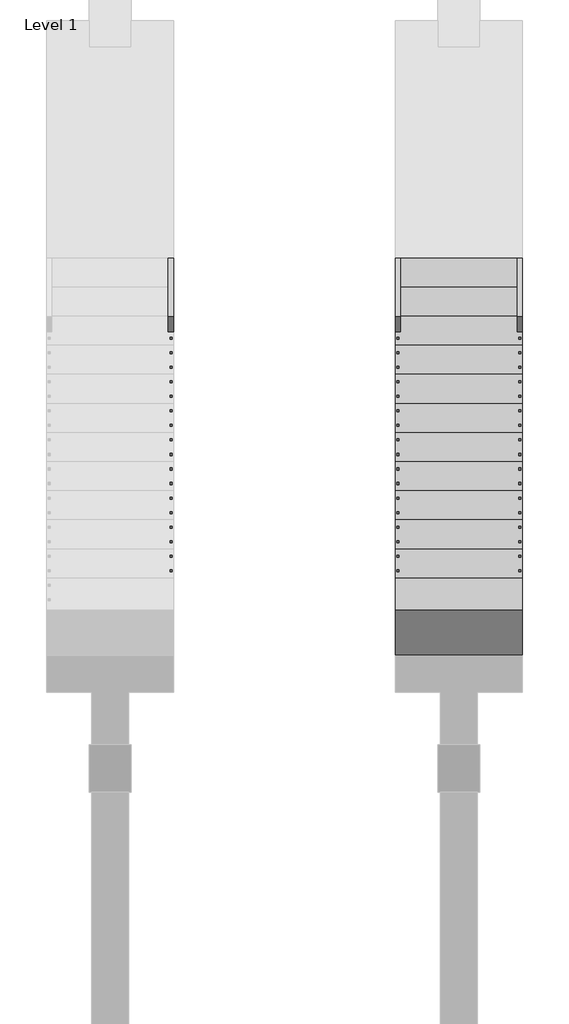
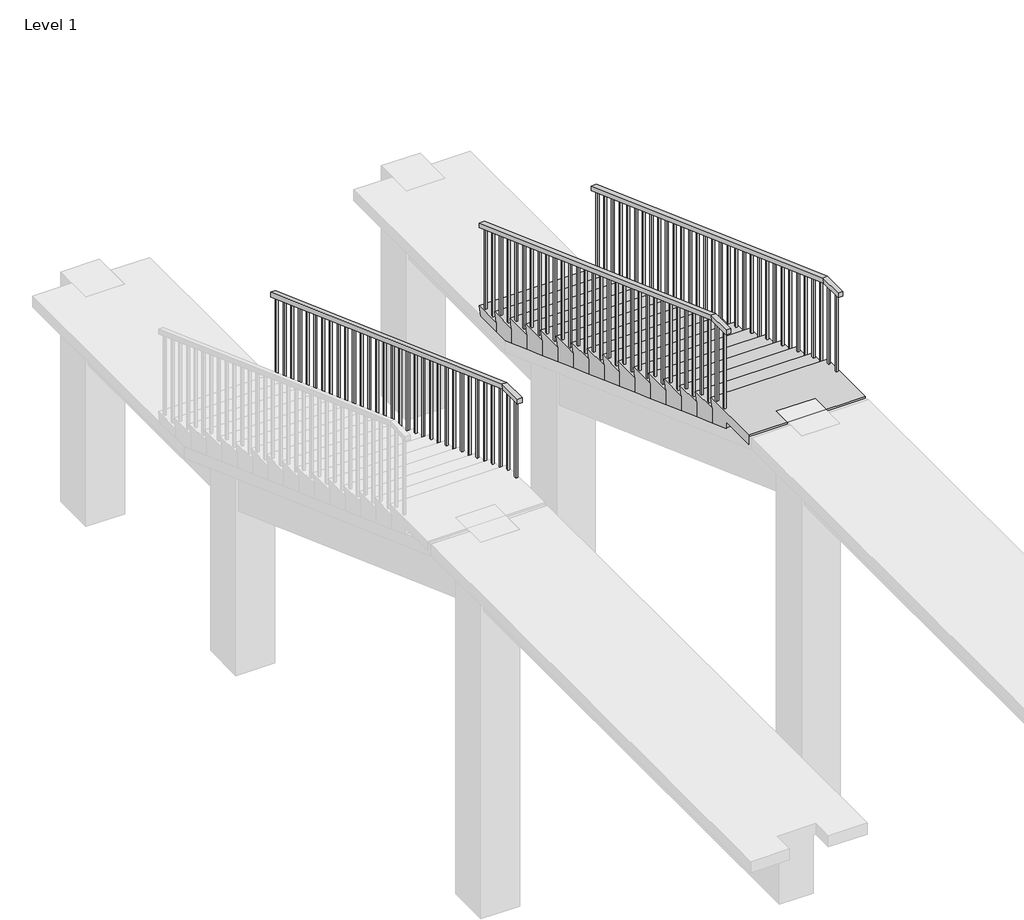
# One storey, part 2 of 2: 3 railings, 1 stair flight.
"""IFC4 building model written with IfcOpenShell, lengths in millimetres."""

from ifc_helpers import new_model, si_unit, frame, origin, place, context, project, spatial, polyline, outline, extrude, faceted_brep, element, save

model = new_model("IFC4")

# Units and contexts
model_context = context("Model", 3, world=origin())
ifc_project = project(units=[si_unit("LENGTHUNIT", "METRE", prefix="MILLI")], contexts=[model_context])

# Site, building, storey
site = spatial("IfcSite", under=ifc_project)
building = spatial("IfcBuilding", under=site)
storey = spatial("IfcBuildingStorey", under=building, Name="Level 1", Elevation=0.0)

# Railings
placement = place(None, origin())
element("IfcRailing", 1, ObjectType="900mm", at=placement, inside=storey, context=model_context, shape_type="SolidModel", body=[
    faceted_brep([(-3859.0267942, 6735.8738053, 1000.0), (-3859.0267942, 6735.8738053, 946.7968186), (-3909.0267942, 6735.8738053, 946.7968186), (-3909.0267942, 6735.8738053, 1000.0), (-3859.0267942, 2610.8738053, 2500.0), (-3859.0267942, 2602.0650564, 2450.0), (-3909.0267942, 2602.0650564, 2450.0), (-3909.0267942, 2610.8738053, 2500.0), (-3859.0267942, 2335.8738053, 2500.0), (-3909.0267942, 2335.8738053, 2500.0), (-3909.0267942, 2335.8738053, 2450.0), (-3859.0267942, 2335.8738053, 2450.0)], [[[0, 1, 2, 3]], [[1, 0, 4, 5]], [[2, 1, 5, 6]], [[3, 2, 6, 7]], [[0, 3, 7, 4]], [[8, 9, 10, 11]], [[5, 4, 8, 11]], [[6, 5, 11, 10]], [[7, 6, 10, 9]], [[4, 7, 9, 8]]]),
    extrude(outline(polyline([(-3894.0267942, 2414.6238053), (-3874.0267942, 2414.6238053), (-3874.0267942, 2394.6238053), (-3894.0267942, 2394.6238053), (-3894.0267942, 2414.6238053)])), frame((0.0, 0.0, 1600.0), z_axis=(0.0, 0.0, 1.0), x_axis=(1.0, 0.0, 0.0)), (0.0, 0.0, 1.0), 850.0),
    extrude(outline(polyline([(-3894.0267942, 2552.1238053), (-3874.0267942, 2552.1238053), (-3874.0267942, 2532.1238053), (-3894.0267942, 2532.1238053), (-3894.0267942, 2552.1238053)])), frame((0.0, 0.0, 1600.0), z_axis=(0.0, 0.0, 1.0), x_axis=(1.0, 0.0, 0.0)), (0.0, 0.0, 1.0), 850.0),
    extrude(outline(polyline([(2689.6238053, 2417.9771109), (2689.6238053, 1500.0), (2669.6238053, 1500.0), (2669.6238053, 2425.3845183), (2689.6238053, 2417.9771109)])), frame((-3894.0267942, 0.0, 0.0), z_axis=(1.0, 0.0, 0.0), x_axis=(0.0, 1.0, 0.0)), (0.0, 0.0, 1.0), 20.0),
    extrude(outline(polyline([(2827.1238053, 2367.9771109), (2827.1238053, 1500.0), (2807.1238053, 1500.0), (2807.1238053, 2375.3845183), (2827.1238053, 2367.9771109)])), frame((-3894.0267942, 0.0, 0.0), z_axis=(1.0, 0.0, 0.0), x_axis=(0.0, 1.0, 0.0)), (0.0, 0.0, 1.0), 20.0),
    extrude(outline(polyline([(2964.6238053, 2317.9771109), (2964.6238053, 1400.0), (2944.6238053, 1400.0), (2944.6238053, 2325.3845183), (2964.6238053, 2317.9771109)])), frame((-3894.0267942, 0.0, 0.0), z_axis=(1.0, 0.0, 0.0), x_axis=(0.0, 1.0, 0.0)), (0.0, 0.0, 1.0), 20.0),
    extrude(outline(polyline([(3102.1238053, 2267.9771109), (3102.1238053, 1400.0), (3082.1238053, 1400.0), (3082.1238053, 2275.3845183), (3102.1238053, 2267.9771109)])), frame((-3894.0267942, 0.0, 0.0), z_axis=(1.0, 0.0, 0.0), x_axis=(0.0, 1.0, 0.0)), (0.0, 0.0, 1.0), 20.0),
    extrude(outline(polyline([(3239.6238053, 2217.9771109), (3239.6238053, 1300.0), (3219.6238053, 1300.0), (3219.6238053, 2225.3845183), (3239.6238053, 2217.9771109)])), frame((-3894.0267942, 0.0, 0.0), z_axis=(1.0, 0.0, 0.0), x_axis=(0.0, 1.0, 0.0)), (0.0, 0.0, 1.0), 20.0),
    extrude(outline(polyline([(3377.1238053, 2167.9771109), (3377.1238053, 1300.0), (3357.1238053, 1300.0), (3357.1238053, 2175.3845183), (3377.1238053, 2167.9771109)])), frame((-3894.0267942, 0.0, 0.0), z_axis=(1.0, 0.0, 0.0), x_axis=(0.0, 1.0, 0.0)), (0.0, 0.0, 1.0), 20.0),
    extrude(outline(polyline([(3514.6238053, 2117.9771109), (3514.6238053, 1200.0), (3494.6238053, 1200.0), (3494.6238053, 2125.3845183), (3514.6238053, 2117.9771109)])), frame((-3894.0267942, 0.0, 0.0), z_axis=(1.0, 0.0, 0.0), x_axis=(0.0, 1.0, 0.0)), (0.0, 0.0, 1.0), 20.0),
    extrude(outline(polyline([(3652.1238053, 2067.9771109), (3652.1238053, 1200.0), (3632.1238053, 1200.0), (3632.1238053, 2075.3845183), (3652.1238053, 2067.9771109)])), frame((-3894.0267942, 0.0, 0.0), z_axis=(1.0, 0.0, 0.0), x_axis=(0.0, 1.0, 0.0)), (0.0, 0.0, 1.0), 20.0),
    extrude(outline(polyline([(3789.6238053, 2017.9771109), (3789.6238053, 1100.0), (3769.6238053, 1100.0), (3769.6238053, 2025.3845183), (3789.6238053, 2017.9771109)])), frame((-3894.0267942, 0.0, 0.0), z_axis=(1.0, 0.0, 0.0), x_axis=(0.0, 1.0, 0.0)), (0.0, 0.0, 1.0), 20.0),
    extrude(outline(polyline([(3927.1238053, 1967.9771109), (3927.1238053, 1100.0), (3907.1238053, 1100.0), (3907.1238053, 1975.3845183), (3927.1238053, 1967.9771109)])), frame((-3894.0267942, 0.0, 0.0), z_axis=(1.0, 0.0, 0.0), x_axis=(0.0, 1.0, 0.0)), (0.0, 0.0, 1.0), 20.0),
    extrude(outline(polyline([(4064.6238053, 1917.9771109), (4064.6238053, 1000.0), (4044.6238053, 1000.0), (4044.6238053, 1925.3845183), (4064.6238053, 1917.9771109)])), frame((-3894.0267942, 0.0, 0.0), z_axis=(1.0, 0.0, 0.0), x_axis=(0.0, 1.0, 0.0)), (0.0, 0.0, 1.0), 20.0),
    extrude(outline(polyline([(4202.1238053, 1867.9771109), (4202.1238053, 1000.0), (4182.1238053, 1000.0), (4182.1238053, 1875.3845183), (4202.1238053, 1867.9771109)])), frame((-3894.0267942, 0.0, 0.0), z_axis=(1.0, 0.0, 0.0), x_axis=(0.0, 1.0, 0.0)), (0.0, 0.0, 1.0), 20.0),
    extrude(outline(polyline([(4339.6238053, 1817.9771109), (4339.6238053, 900.0), (4319.6238053, 900.0), (4319.6238053, 1825.3845183), (4339.6238053, 1817.9771109)])), frame((-3894.0267942, 0.0, 0.0), z_axis=(1.0, 0.0, 0.0), x_axis=(0.0, 1.0, 0.0)), (0.0, 0.0, 1.0), 20.0),
    extrude(outline(polyline([(4477.1238053, 1767.9771109), (4477.1238053, 900.0), (4457.1238053, 900.0), (4457.1238053, 1775.3845183), (4477.1238053, 1767.9771109)])), frame((-3894.0267942, 0.0, 0.0), z_axis=(1.0, 0.0, 0.0), x_axis=(0.0, 1.0, 0.0)), (0.0, 0.0, 1.0), 20.0),
    extrude(outline(polyline([(4614.6238053, 1717.9771109), (4614.6238053, 800.0), (4594.6238053, 800.0), (4594.6238053, 1725.3845183), (4614.6238053, 1717.9771109)])), frame((-3894.0267942, 0.0, 0.0), z_axis=(1.0, 0.0, 0.0), x_axis=(0.0, 1.0, 0.0)), (0.0, 0.0, 1.0), 20.0),
    extrude(outline(polyline([(4752.1238053, 1667.9771109), (4752.1238053, 800.0), (4732.1238053, 800.0), (4732.1238053, 1675.3845183), (4752.1238053, 1667.9771109)])), frame((-3894.0267942, 0.0, 0.0), z_axis=(1.0, 0.0, 0.0), x_axis=(0.0, 1.0, 0.0)), (0.0, 0.0, 1.0), 20.0),
    extrude(outline(polyline([(4889.6238053, 1617.9771109), (4889.6238053, 700.0), (4869.6238053, 700.0), (4869.6238053, 1625.3845183), (4889.6238053, 1617.9771109)])), frame((-3894.0267942, 0.0, 0.0), z_axis=(1.0, 0.0, 0.0), x_axis=(0.0, 1.0, 0.0)), (0.0, 0.0, 1.0), 20.0),
    extrude(outline(polyline([(5027.1238053, 1567.9771109), (5027.1238053, 700.0), (5007.1238053, 700.0), (5007.1238053, 1575.3845183), (5027.1238053, 1567.9771109)])), frame((-3894.0267942, 0.0, 0.0), z_axis=(1.0, 0.0, 0.0), x_axis=(0.0, 1.0, 0.0)), (0.0, 0.0, 1.0), 20.0),
    extrude(outline(polyline([(5164.6238053, 1517.9771109), (5164.6238053, 600.0), (5144.6238053, 600.0), (5144.6238053, 1525.3845183), (5164.6238053, 1517.9771109)])), frame((-3894.0267942, 0.0, 0.0), z_axis=(1.0, 0.0, 0.0), x_axis=(0.0, 1.0, 0.0)), (0.0, 0.0, 1.0), 20.0),
    extrude(outline(polyline([(5302.1238053, 1467.9771109), (5302.1238053, 600.0), (5282.1238053, 600.0), (5282.1238053, 1475.3845183), (5302.1238053, 1467.9771109)])), frame((-3894.0267942, 0.0, 0.0), z_axis=(1.0, 0.0, 0.0), x_axis=(0.0, 1.0, 0.0)), (0.0, 0.0, 1.0), 20.0),
    extrude(outline(polyline([(5439.6238053, 1417.9771109), (5439.6238053, 500.0), (5419.6238053, 500.0), (5419.6238053, 1425.3845183), (5439.6238053, 1417.9771109)])), frame((-3894.0267942, 0.0, 0.0), z_axis=(1.0, 0.0, 0.0), x_axis=(0.0, 1.0, 0.0)), (0.0, 0.0, 1.0), 20.0),
    extrude(outline(polyline([(5577.1238053, 1367.9771109), (5577.1238053, 500.0), (5557.1238053, 500.0), (5557.1238053, 1375.3845183), (5577.1238053, 1367.9771109)])), frame((-3894.0267942, 0.0, 0.0), z_axis=(1.0, 0.0, 0.0), x_axis=(0.0, 1.0, 0.0)), (0.0, 0.0, 1.0), 20.0),
    extrude(outline(polyline([(5714.6238053, 1317.9771109), (5714.6238053, 400.0), (5694.6238053, 400.0), (5694.6238053, 1325.3845183), (5714.6238053, 1317.9771109)])), frame((-3894.0267942, 0.0, 0.0), z_axis=(1.0, 0.0, 0.0), x_axis=(0.0, 1.0, 0.0)), (0.0, 0.0, 1.0), 20.0),
    extrude(outline(polyline([(5852.1238053, 1267.9771109), (5852.1238053, 400.0), (5832.1238053, 400.0), (5832.1238053, 1275.3845183), (5852.1238053, 1267.9771109)])), frame((-3894.0267942, 0.0, 0.0), z_axis=(1.0, 0.0, 0.0), x_axis=(0.0, 1.0, 0.0)), (0.0, 0.0, 1.0), 20.0),
    extrude(outline(polyline([(5989.6238053, 1217.9771109), (5989.6238053, 300.0), (5969.6238053, 300.0), (5969.6238053, 1225.3845183), (5989.6238053, 1217.9771109)])), frame((-3894.0267942, 0.0, 0.0), z_axis=(1.0, 0.0, 0.0), x_axis=(0.0, 1.0, 0.0)), (0.0, 0.0, 1.0), 20.0),
    extrude(outline(polyline([(6127.1238053, 1167.9771109), (6127.1238053, 300.0), (6107.1238053, 300.0), (6107.1238053, 1175.3845183), (6127.1238053, 1167.9771109)])), frame((-3894.0267942, 0.0, 0.0), z_axis=(1.0, 0.0, 0.0), x_axis=(0.0, 1.0, 0.0)), (0.0, 0.0, 1.0), 20.0),
    extrude(outline(polyline([(6264.6238053, 1117.9771109), (6264.6238053, 200.0), (6244.6238053, 200.0), (6244.6238053, 1125.3845183), (6264.6238053, 1117.9771109)])), frame((-3894.0267942, 0.0, 0.0), z_axis=(1.0, 0.0, 0.0), x_axis=(0.0, 1.0, 0.0)), (0.0, 0.0, 1.0), 20.0),
    extrude(outline(polyline([(6402.1238053, 1067.9771109), (6402.1238053, 200.0), (6382.1238053, 200.0), (6382.1238053, 1075.3845183), (6402.1238053, 1067.9771109)])), frame((-3894.0267942, 0.0, 0.0), z_axis=(1.0, 0.0, 0.0), x_axis=(0.0, 1.0, 0.0)), (0.0, 0.0, 1.0), 20.0),
    extrude(outline(polyline([(6539.6238053, 1017.9771109), (6539.6238053, 100.0), (6519.6238053, 100.0), (6519.6238053, 1025.3845183), (6539.6238053, 1017.9771109)])), frame((-3894.0267942, 0.0, 0.0), z_axis=(1.0, 0.0, 0.0), x_axis=(0.0, 1.0, 0.0)), (0.0, 0.0, 1.0), 20.0),
    extrude(outline(polyline([(6677.1238053, 967.9771109), (6677.1238053, 100.0), (6657.1238053, 100.0), (6657.1238053, 975.3845183), (6677.1238053, 967.9771109)])), frame((-3894.0267942, 0.0, 0.0), z_axis=(1.0, 0.0, 0.0), x_axis=(0.0, 1.0, 0.0)), (0.0, 0.0, 1.0), 20.0),
])
element("IfcRailing", 2, ObjectType="900mm", at=placement, inside=storey, context=model_context, shape_type="SolidModel", body=[
    faceted_brep([(-2706.8056398, 6735.8738053, 1000.0), (-2706.8056398, 6735.8738053, 946.7968186), (-2756.8056398, 6735.8738053, 946.7968186), (-2756.8056398, 6735.8738053, 1000.0), (-2706.8056398, 2610.8738053, 2500.0), (-2706.8056398, 2602.0650564, 2450.0), (-2756.8056398, 2602.0650564, 2450.0), (-2756.8056398, 2610.8738053, 2500.0), (-2706.8056398, 2335.8738053, 2500.0), (-2756.8056398, 2335.8738053, 2500.0), (-2756.8056398, 2335.8738053, 2450.0), (-2706.8056398, 2335.8738053, 2450.0)], [[[0, 1, 2, 3]], [[1, 0, 4, 5]], [[2, 1, 5, 6]], [[3, 2, 6, 7]], [[0, 3, 7, 4]], [[8, 9, 10, 11]], [[5, 4, 8, 11]], [[6, 5, 11, 10]], [[7, 6, 10, 9]], [[4, 7, 9, 8]]]),
    extrude(outline(polyline([(-2721.8056398, 2414.6238053), (-2721.8056398, 2394.6238053), (-2741.8056398, 2394.6238053), (-2741.8056398, 2414.6238053), (-2721.8056398, 2414.6238053)])), frame((0.0, 0.0, 1600.0), z_axis=(0.0, 0.0, 1.0), x_axis=(1.0, 0.0, 0.0)), (0.0, 0.0, 1.0), 850.0),
    extrude(outline(polyline([(-2721.8056398, 2552.1238053), (-2721.8056398, 2532.1238053), (-2741.8056398, 2532.1238053), (-2741.8056398, 2552.1238053), (-2721.8056398, 2552.1238053)])), frame((0.0, 0.0, 1600.0), z_axis=(0.0, 0.0, 1.0), x_axis=(1.0, 0.0, 0.0)), (0.0, 0.0, 1.0), 850.0),
    extrude(outline(polyline([(2689.6238053, 1500.0), (2669.6238053, 1500.0), (2669.6238053, 2425.3845183), (2689.6238053, 2417.9771109), (2689.6238053, 1500.0)])), frame((-2741.8056398, 0.0, 0.0), z_axis=(1.0, 0.0, 0.0), x_axis=(0.0, 1.0, 0.0)), (0.0, 0.0, 1.0), 20.0),
    extrude(outline(polyline([(2827.1238053, 1500.0), (2807.1238053, 1500.0), (2807.1238053, 2375.3845183), (2827.1238053, 2367.9771109), (2827.1238053, 1500.0)])), frame((-2741.8056398, 0.0, 0.0), z_axis=(1.0, 0.0, 0.0), x_axis=(0.0, 1.0, 0.0)), (0.0, 0.0, 1.0), 20.0),
    extrude(outline(polyline([(2964.6238053, 1400.0), (2944.6238053, 1400.0), (2944.6238053, 2325.3845183), (2964.6238053, 2317.9771109), (2964.6238053, 1400.0)])), frame((-2741.8056398, 0.0, 0.0), z_axis=(1.0, 0.0, 0.0), x_axis=(0.0, 1.0, 0.0)), (0.0, 0.0, 1.0), 20.0),
    extrude(outline(polyline([(3102.1238053, 1400.0), (3082.1238053, 1400.0), (3082.1238053, 2275.3845183), (3102.1238053, 2267.9771109), (3102.1238053, 1400.0)])), frame((-2741.8056398, 0.0, 0.0), z_axis=(1.0, 0.0, 0.0), x_axis=(0.0, 1.0, 0.0)), (0.0, 0.0, 1.0), 20.0),
    extrude(outline(polyline([(3239.6238053, 1300.0), (3219.6238053, 1300.0), (3219.6238053, 2225.3845183), (3239.6238053, 2217.9771109), (3239.6238053, 1300.0)])), frame((-2741.8056398, 0.0, 0.0), z_axis=(1.0, 0.0, 0.0), x_axis=(0.0, 1.0, 0.0)), (0.0, 0.0, 1.0), 20.0),
    extrude(outline(polyline([(3377.1238053, 1300.0), (3357.1238053, 1300.0), (3357.1238053, 2175.3845183), (3377.1238053, 2167.9771109), (3377.1238053, 1300.0)])), frame((-2741.8056398, 0.0, 0.0), z_axis=(1.0, 0.0, 0.0), x_axis=(0.0, 1.0, 0.0)), (0.0, 0.0, 1.0), 20.0),
    extrude(outline(polyline([(3514.6238053, 1200.0), (3494.6238053, 1200.0), (3494.6238053, 2125.3845183), (3514.6238053, 2117.9771109), (3514.6238053, 1200.0)])), frame((-2741.8056398, 0.0, 0.0), z_axis=(1.0, 0.0, 0.0), x_axis=(0.0, 1.0, 0.0)), (0.0, 0.0, 1.0), 20.0),
    extrude(outline(polyline([(3652.1238053, 1200.0), (3632.1238053, 1200.0), (3632.1238053, 2075.3845183), (3652.1238053, 2067.9771109), (3652.1238053, 1200.0)])), frame((-2741.8056398, 0.0, 0.0), z_axis=(1.0, 0.0, 0.0), x_axis=(0.0, 1.0, 0.0)), (0.0, 0.0, 1.0), 20.0),
    extrude(outline(polyline([(3789.6238053, 1100.0), (3769.6238053, 1100.0), (3769.6238053, 2025.3845183), (3789.6238053, 2017.9771109), (3789.6238053, 1100.0)])), frame((-2741.8056398, 0.0, 0.0), z_axis=(1.0, 0.0, 0.0), x_axis=(0.0, 1.0, 0.0)), (0.0, 0.0, 1.0), 20.0),
    extrude(outline(polyline([(3927.1238053, 1100.0), (3907.1238053, 1100.0), (3907.1238053, 1975.3845183), (3927.1238053, 1967.9771109), (3927.1238053, 1100.0)])), frame((-2741.8056398, 0.0, 0.0), z_axis=(1.0, 0.0, 0.0), x_axis=(0.0, 1.0, 0.0)), (0.0, 0.0, 1.0), 20.0),
    extrude(outline(polyline([(4064.6238053, 1000.0), (4044.6238053, 1000.0), (4044.6238053, 1925.3845183), (4064.6238053, 1917.9771109), (4064.6238053, 1000.0)])), frame((-2741.8056398, 0.0, 0.0), z_axis=(1.0, 0.0, 0.0), x_axis=(0.0, 1.0, 0.0)), (0.0, 0.0, 1.0), 20.0),
    extrude(outline(polyline([(4202.1238053, 1000.0), (4182.1238053, 1000.0), (4182.1238053, 1875.3845183), (4202.1238053, 1867.9771109), (4202.1238053, 1000.0)])), frame((-2741.8056398, 0.0, 0.0), z_axis=(1.0, 0.0, 0.0), x_axis=(0.0, 1.0, 0.0)), (0.0, 0.0, 1.0), 20.0),
    extrude(outline(polyline([(4339.6238053, 900.0), (4319.6238053, 900.0), (4319.6238053, 1825.3845183), (4339.6238053, 1817.9771109), (4339.6238053, 900.0)])), frame((-2741.8056398, 0.0, 0.0), z_axis=(1.0, 0.0, 0.0), x_axis=(0.0, 1.0, 0.0)), (0.0, 0.0, 1.0), 20.0),
    extrude(outline(polyline([(4477.1238053, 900.0), (4457.1238053, 900.0), (4457.1238053, 1775.3845183), (4477.1238053, 1767.9771109), (4477.1238053, 900.0)])), frame((-2741.8056398, 0.0, 0.0), z_axis=(1.0, 0.0, 0.0), x_axis=(0.0, 1.0, 0.0)), (0.0, 0.0, 1.0), 20.0),
    extrude(outline(polyline([(4614.6238053, 800.0), (4594.6238053, 800.0), (4594.6238053, 1725.3845183), (4614.6238053, 1717.9771109), (4614.6238053, 800.0)])), frame((-2741.8056398, 0.0, 0.0), z_axis=(1.0, 0.0, 0.0), x_axis=(0.0, 1.0, 0.0)), (0.0, 0.0, 1.0), 20.0),
    extrude(outline(polyline([(4752.1238053, 800.0), (4732.1238053, 800.0), (4732.1238053, 1675.3845183), (4752.1238053, 1667.9771109), (4752.1238053, 800.0)])), frame((-2741.8056398, 0.0, 0.0), z_axis=(1.0, 0.0, 0.0), x_axis=(0.0, 1.0, 0.0)), (0.0, 0.0, 1.0), 20.0),
    extrude(outline(polyline([(4889.6238053, 700.0), (4869.6238053, 700.0), (4869.6238053, 1625.3845183), (4889.6238053, 1617.9771109), (4889.6238053, 700.0)])), frame((-2741.8056398, 0.0, 0.0), z_axis=(1.0, 0.0, 0.0), x_axis=(0.0, 1.0, 0.0)), (0.0, 0.0, 1.0), 20.0),
    extrude(outline(polyline([(5027.1238053, 700.0), (5007.1238053, 700.0), (5007.1238053, 1575.3845183), (5027.1238053, 1567.9771109), (5027.1238053, 700.0)])), frame((-2741.8056398, 0.0, 0.0), z_axis=(1.0, 0.0, 0.0), x_axis=(0.0, 1.0, 0.0)), (0.0, 0.0, 1.0), 20.0),
    extrude(outline(polyline([(5164.6238053, 600.0), (5144.6238053, 600.0), (5144.6238053, 1525.3845183), (5164.6238053, 1517.9771109), (5164.6238053, 600.0)])), frame((-2741.8056398, 0.0, 0.0), z_axis=(1.0, 0.0, 0.0), x_axis=(0.0, 1.0, 0.0)), (0.0, 0.0, 1.0), 20.0),
    extrude(outline(polyline([(5302.1238053, 600.0), (5282.1238053, 600.0), (5282.1238053, 1475.3845183), (5302.1238053, 1467.9771109), (5302.1238053, 600.0)])), frame((-2741.8056398, 0.0, 0.0), z_axis=(1.0, 0.0, 0.0), x_axis=(0.0, 1.0, 0.0)), (0.0, 0.0, 1.0), 20.0),
    extrude(outline(polyline([(5439.6238053, 500.0), (5419.6238053, 500.0), (5419.6238053, 1425.3845183), (5439.6238053, 1417.9771109), (5439.6238053, 500.0)])), frame((-2741.8056398, 0.0, 0.0), z_axis=(1.0, 0.0, 0.0), x_axis=(0.0, 1.0, 0.0)), (0.0, 0.0, 1.0), 20.0),
    extrude(outline(polyline([(5577.1238053, 500.0), (5557.1238053, 500.0), (5557.1238053, 1375.3845183), (5577.1238053, 1367.9771109), (5577.1238053, 500.0)])), frame((-2741.8056398, 0.0, 0.0), z_axis=(1.0, 0.0, 0.0), x_axis=(0.0, 1.0, 0.0)), (0.0, 0.0, 1.0), 20.0),
    extrude(outline(polyline([(5714.6238053, 400.0), (5694.6238053, 400.0), (5694.6238053, 1325.3845183), (5714.6238053, 1317.9771109), (5714.6238053, 400.0)])), frame((-2741.8056398, 0.0, 0.0), z_axis=(1.0, 0.0, 0.0), x_axis=(0.0, 1.0, 0.0)), (0.0, 0.0, 1.0), 20.0),
    extrude(outline(polyline([(5852.1238053, 400.0), (5832.1238053, 400.0), (5832.1238053, 1275.3845183), (5852.1238053, 1267.9771109), (5852.1238053, 400.0)])), frame((-2741.8056398, 0.0, 0.0), z_axis=(1.0, 0.0, 0.0), x_axis=(0.0, 1.0, 0.0)), (0.0, 0.0, 1.0), 20.0),
    extrude(outline(polyline([(5989.6238053, 300.0), (5969.6238053, 300.0), (5969.6238053, 1225.3845183), (5989.6238053, 1217.9771109), (5989.6238053, 300.0)])), frame((-2741.8056398, 0.0, 0.0), z_axis=(1.0, 0.0, 0.0), x_axis=(0.0, 1.0, 0.0)), (0.0, 0.0, 1.0), 20.0),
    extrude(outline(polyline([(6127.1238053, 300.0), (6107.1238053, 300.0), (6107.1238053, 1175.3845183), (6127.1238053, 1167.9771109), (6127.1238053, 300.0)])), frame((-2741.8056398, 0.0, 0.0), z_axis=(1.0, 0.0, 0.0), x_axis=(0.0, 1.0, 0.0)), (0.0, 0.0, 1.0), 20.0),
    extrude(outline(polyline([(6264.6238053, 200.0), (6244.6238053, 200.0), (6244.6238053, 1125.3845183), (6264.6238053, 1117.9771109), (6264.6238053, 200.0)])), frame((-2741.8056398, 0.0, 0.0), z_axis=(1.0, 0.0, 0.0), x_axis=(0.0, 1.0, 0.0)), (0.0, 0.0, 1.0), 20.0),
    extrude(outline(polyline([(6402.1238053, 200.0), (6382.1238053, 200.0), (6382.1238053, 1075.3845183), (6402.1238053, 1067.9771109), (6402.1238053, 200.0)])), frame((-2741.8056398, 0.0, 0.0), z_axis=(1.0, 0.0, 0.0), x_axis=(0.0, 1.0, 0.0)), (0.0, 0.0, 1.0), 20.0),
    extrude(outline(polyline([(6539.6238053, 100.0), (6519.6238053, 100.0), (6519.6238053, 1025.3845183), (6539.6238053, 1017.9771109), (6539.6238053, 100.0)])), frame((-2741.8056398, 0.0, 0.0), z_axis=(1.0, 0.0, 0.0), x_axis=(0.0, 1.0, 0.0)), (0.0, 0.0, 1.0), 20.0),
    extrude(outline(polyline([(6677.1238053, 100.0), (6657.1238053, 100.0), (6657.1238053, 975.3845183), (6677.1238053, 967.9771109), (6677.1238053, 100.0)])), frame((-2741.8056398, 0.0, 0.0), z_axis=(1.0, 0.0, 0.0), x_axis=(0.0, 1.0, 0.0)), (0.0, 0.0, 1.0), 20.0),
])
element("IfcRailing", 3, ObjectType="900mm", at=placement, inside=storey, context=model_context, shape_type="SolidModel", body=[
    faceted_brep([(-6006.8056398, 6735.8738053, 1000.0), (-6006.8056398, 6735.8738053, 946.7968186), (-6056.8056398, 6735.8738053, 946.7968186), (-6056.8056398, 6735.8738053, 1000.0), (-6006.8056398, 2610.8738053, 2500.0), (-6006.8056398, 2602.0650564, 2450.0), (-6056.8056398, 2602.0650564, 2450.0), (-6056.8056398, 2610.8738053, 2500.0), (-6006.8056398, 2335.8738053, 2500.0), (-6056.8056398, 2335.8738053, 2500.0), (-6056.8056398, 2335.8738053, 2450.0), (-6006.8056398, 2335.8738053, 2450.0)], [[[0, 1, 2, 3]], [[1, 0, 4, 5]], [[2, 1, 5, 6]], [[3, 2, 6, 7]], [[0, 3, 7, 4]], [[8, 9, 10, 11]], [[5, 4, 8, 11]], [[6, 5, 11, 10]], [[7, 6, 10, 9]], [[4, 7, 9, 8]]]),
    extrude(outline(polyline([(-6021.8056398, 2414.6238053), (-6021.8056398, 2394.6238053), (-6041.8056398, 2394.6238053), (-6041.8056398, 2414.6238053), (-6021.8056398, 2414.6238053)])), frame((0.0, 0.0, 1600.0), z_axis=(0.0, 0.0, 1.0), x_axis=(1.0, 0.0, 0.0)), (0.0, 0.0, 1.0), 850.0),
    extrude(outline(polyline([(-6021.8056398, 2552.1238053), (-6021.8056398, 2532.1238053), (-6041.8056398, 2532.1238053), (-6041.8056398, 2552.1238053), (-6021.8056398, 2552.1238053)])), frame((0.0, 0.0, 1600.0), z_axis=(0.0, 0.0, 1.0), x_axis=(1.0, 0.0, 0.0)), (0.0, 0.0, 1.0), 850.0),
    extrude(outline(polyline([(2689.6238053, 1500.0), (2669.6238053, 1500.0), (2669.6238053, 2425.4331822), (2689.6238053, 2418.160455), (2689.6238053, 1500.0)])), frame((-6041.8056398, 0.0, 0.0), z_axis=(1.0, 0.0, 0.0), x_axis=(0.0, 1.0, 0.0)), (0.0, 0.0, 1.0), 20.0),
    extrude(outline(polyline([(2827.1238053, 1500.0), (2807.1238053, 1500.0), (2807.1238053, 2375.4331822), (2827.1238053, 2368.160455), (2827.1238053, 1500.0)])), frame((-6041.8056398, 0.0, 0.0), z_axis=(1.0, 0.0, 0.0), x_axis=(0.0, 1.0, 0.0)), (0.0, 0.0, 1.0), 20.0),
    extrude(outline(polyline([(2964.6238053, 1400.0), (2944.6238053, 1400.0), (2944.6238053, 2325.4331822), (2964.6238053, 2318.160455), (2964.6238053, 1400.0)])), frame((-6041.8056398, 0.0, 0.0), z_axis=(1.0, 0.0, 0.0), x_axis=(0.0, 1.0, 0.0)), (0.0, 0.0, 1.0), 20.0),
    extrude(outline(polyline([(3102.1238053, 1400.0), (3082.1238053, 1400.0), (3082.1238053, 2275.4331822), (3102.1238053, 2268.160455), (3102.1238053, 1400.0)])), frame((-6041.8056398, 0.0, 0.0), z_axis=(1.0, 0.0, 0.0), x_axis=(0.0, 1.0, 0.0)), (0.0, 0.0, 1.0), 20.0),
    extrude(outline(polyline([(3239.6238053, 1300.0), (3219.6238053, 1300.0), (3219.6238053, 2225.4331822), (3239.6238053, 2218.160455), (3239.6238053, 1300.0)])), frame((-6041.8056398, 0.0, 0.0), z_axis=(1.0, 0.0, 0.0), x_axis=(0.0, 1.0, 0.0)), (0.0, 0.0, 1.0), 20.0),
    extrude(outline(polyline([(3377.1238053, 1300.0), (3357.1238053, 1300.0), (3357.1238053, 2175.4331822), (3377.1238053, 2168.160455), (3377.1238053, 1300.0)])), frame((-6041.8056398, 0.0, 0.0), z_axis=(1.0, 0.0, 0.0), x_axis=(0.0, 1.0, 0.0)), (0.0, 0.0, 1.0), 20.0),
    extrude(outline(polyline([(3514.6238053, 1200.0), (3494.6238053, 1200.0), (3494.6238053, 2125.4331822), (3514.6238053, 2118.160455), (3514.6238053, 1200.0)])), frame((-6041.8056398, 0.0, 0.0), z_axis=(1.0, 0.0, 0.0), x_axis=(0.0, 1.0, 0.0)), (0.0, 0.0, 1.0), 20.0),
    extrude(outline(polyline([(3652.1238053, 1200.0), (3632.1238053, 1200.0), (3632.1238053, 2075.4331822), (3652.1238053, 2068.160455), (3652.1238053, 1200.0)])), frame((-6041.8056398, 0.0, 0.0), z_axis=(1.0, 0.0, 0.0), x_axis=(0.0, 1.0, 0.0)), (0.0, 0.0, 1.0), 20.0),
    extrude(outline(polyline([(3789.6238053, 1100.0), (3769.6238053, 1100.0), (3769.6238053, 2025.4331822), (3789.6238053, 2018.160455), (3789.6238053, 1100.0)])), frame((-6041.8056398, 0.0, 0.0), z_axis=(1.0, 0.0, 0.0), x_axis=(0.0, 1.0, 0.0)), (0.0, 0.0, 1.0), 20.0),
    extrude(outline(polyline([(3927.1238053, 1100.0), (3907.1238053, 1100.0), (3907.1238053, 1975.4331822), (3927.1238053, 1968.160455), (3927.1238053, 1100.0)])), frame((-6041.8056398, 0.0, 0.0), z_axis=(1.0, 0.0, 0.0), x_axis=(0.0, 1.0, 0.0)), (0.0, 0.0, 1.0), 20.0),
    extrude(outline(polyline([(4064.6238053, 1000.0), (4044.6238053, 1000.0), (4044.6238053, 1925.4331822), (4064.6238053, 1918.160455), (4064.6238053, 1000.0)])), frame((-6041.8056398, 0.0, 0.0), z_axis=(1.0, 0.0, 0.0), x_axis=(0.0, 1.0, 0.0)), (0.0, 0.0, 1.0), 20.0),
    extrude(outline(polyline([(4202.1238053, 1000.0), (4182.1238053, 1000.0), (4182.1238053, 1875.4331822), (4202.1238053, 1868.160455), (4202.1238053, 1000.0)])), frame((-6041.8056398, 0.0, 0.0), z_axis=(1.0, 0.0, 0.0), x_axis=(0.0, 1.0, 0.0)), (0.0, 0.0, 1.0), 20.0),
    extrude(outline(polyline([(4339.6238053, 900.0), (4319.6238053, 900.0), (4319.6238053, 1825.4331822), (4339.6238053, 1818.160455), (4339.6238053, 900.0)])), frame((-6041.8056398, 0.0, 0.0), z_axis=(1.0, 0.0, 0.0), x_axis=(0.0, 1.0, 0.0)), (0.0, 0.0, 1.0), 20.0),
    extrude(outline(polyline([(4477.1238053, 900.0), (4457.1238053, 900.0), (4457.1238053, 1775.4331822), (4477.1238053, 1768.160455), (4477.1238053, 900.0)])), frame((-6041.8056398, 0.0, 0.0), z_axis=(1.0, 0.0, 0.0), x_axis=(0.0, 1.0, 0.0)), (0.0, 0.0, 1.0), 20.0),
    extrude(outline(polyline([(4614.6238053, 800.0), (4594.6238053, 800.0), (4594.6238053, 1725.4331822), (4614.6238053, 1718.160455), (4614.6238053, 800.0)])), frame((-6041.8056398, 0.0, 0.0), z_axis=(1.0, 0.0, 0.0), x_axis=(0.0, 1.0, 0.0)), (0.0, 0.0, 1.0), 20.0),
    extrude(outline(polyline([(4752.1238053, 800.0), (4732.1238053, 800.0), (4732.1238053, 1675.4331822), (4752.1238053, 1668.160455), (4752.1238053, 800.0)])), frame((-6041.8056398, 0.0, 0.0), z_axis=(1.0, 0.0, 0.0), x_axis=(0.0, 1.0, 0.0)), (0.0, 0.0, 1.0), 20.0),
    extrude(outline(polyline([(4889.6238053, 700.0), (4869.6238053, 700.0), (4869.6238053, 1625.4331822), (4889.6238053, 1618.160455), (4889.6238053, 700.0)])), frame((-6041.8056398, 0.0, 0.0), z_axis=(1.0, 0.0, 0.0), x_axis=(0.0, 1.0, 0.0)), (0.0, 0.0, 1.0), 20.0),
    extrude(outline(polyline([(5027.1238053, 700.0), (5007.1238053, 700.0), (5007.1238053, 1575.4331822), (5027.1238053, 1568.160455), (5027.1238053, 700.0)])), frame((-6041.8056398, 0.0, 0.0), z_axis=(1.0, 0.0, 0.0), x_axis=(0.0, 1.0, 0.0)), (0.0, 0.0, 1.0), 20.0),
    extrude(outline(polyline([(5164.6238053, 600.0), (5144.6238053, 600.0), (5144.6238053, 1525.4331822), (5164.6238053, 1518.160455), (5164.6238053, 600.0)])), frame((-6041.8056398, 0.0, 0.0), z_axis=(1.0, 0.0, 0.0), x_axis=(0.0, 1.0, 0.0)), (0.0, 0.0, 1.0), 20.0),
    extrude(outline(polyline([(5302.1238053, 600.0), (5282.1238053, 600.0), (5282.1238053, 1475.4331822), (5302.1238053, 1468.160455), (5302.1238053, 600.0)])), frame((-6041.8056398, 0.0, 0.0), z_axis=(1.0, 0.0, 0.0), x_axis=(0.0, 1.0, 0.0)), (0.0, 0.0, 1.0), 20.0),
    extrude(outline(polyline([(5439.6238053, 500.0), (5419.6238053, 500.0), (5419.6238053, 1425.4331822), (5439.6238053, 1418.160455), (5439.6238053, 500.0)])), frame((-6041.8056398, 0.0, 0.0), z_axis=(1.0, 0.0, 0.0), x_axis=(0.0, 1.0, 0.0)), (0.0, 0.0, 1.0), 20.0),
    extrude(outline(polyline([(5577.1238053, 500.0), (5557.1238053, 500.0), (5557.1238053, 1375.4331822), (5577.1238053, 1368.160455), (5577.1238053, 500.0)])), frame((-6041.8056398, 0.0, 0.0), z_axis=(1.0, 0.0, 0.0), x_axis=(0.0, 1.0, 0.0)), (0.0, 0.0, 1.0), 20.0),
    extrude(outline(polyline([(5714.6238053, 400.0), (5694.6238053, 400.0), (5694.6238053, 1325.4331822), (5714.6238053, 1318.160455), (5714.6238053, 400.0)])), frame((-6041.8056398, 0.0, 0.0), z_axis=(1.0, 0.0, 0.0), x_axis=(0.0, 1.0, 0.0)), (0.0, 0.0, 1.0), 20.0),
    extrude(outline(polyline([(5852.1238053, 400.0), (5832.1238053, 400.0), (5832.1238053, 1275.4331822), (5852.1238053, 1268.160455), (5852.1238053, 400.0)])), frame((-6041.8056398, 0.0, 0.0), z_axis=(1.0, 0.0, 0.0), x_axis=(0.0, 1.0, 0.0)), (0.0, 0.0, 1.0), 20.0),
    extrude(outline(polyline([(5989.6238053, 300.0), (5969.6238053, 300.0), (5969.6238053, 1225.4331822), (5989.6238053, 1218.160455), (5989.6238053, 300.0)])), frame((-6041.8056398, 0.0, 0.0), z_axis=(1.0, 0.0, 0.0), x_axis=(0.0, 1.0, 0.0)), (0.0, 0.0, 1.0), 20.0),
    extrude(outline(polyline([(6127.1238053, 300.0), (6107.1238053, 300.0), (6107.1238053, 1175.4331822), (6127.1238053, 1168.160455), (6127.1238053, 300.0)])), frame((-6041.8056398, 0.0, 0.0), z_axis=(1.0, 0.0, 0.0), x_axis=(0.0, 1.0, 0.0)), (0.0, 0.0, 1.0), 20.0),
    extrude(outline(polyline([(6264.6238053, 200.0), (6244.6238053, 200.0), (6244.6238053, 1125.4331822), (6264.6238053, 1118.160455), (6264.6238053, 200.0)])), frame((-6041.8056398, 0.0, 0.0), z_axis=(1.0, 0.0, 0.0), x_axis=(0.0, 1.0, 0.0)), (0.0, 0.0, 1.0), 20.0),
    extrude(outline(polyline([(6402.1238053, 200.0), (6382.1238053, 200.0), (6382.1238053, 1075.4331822), (6402.1238053, 1068.160455), (6402.1238053, 200.0)])), frame((-6041.8056398, 0.0, 0.0), z_axis=(1.0, 0.0, 0.0), x_axis=(0.0, 1.0, 0.0)), (0.0, 0.0, 1.0), 20.0),
    extrude(outline(polyline([(6539.6238053, 100.0), (6519.6238053, 100.0), (6519.6238053, 1025.4331822), (6539.6238053, 1018.160455), (6539.6238053, 100.0)])), frame((-6041.8056398, 0.0, 0.0), z_axis=(1.0, 0.0, 0.0), x_axis=(0.0, 1.0, 0.0)), (0.0, 0.0, 1.0), 20.0),
    extrude(outline(polyline([(6677.1238053, 100.0), (6657.1238053, 100.0), (6657.1238053, 975.4331822), (6677.1238053, 968.160455), (6677.1238053, 100.0)])), frame((-6041.8056398, 0.0, 0.0), z_axis=(1.0, 0.0, 0.0), x_axis=(0.0, 1.0, 0.0)), (0.0, 0.0, 1.0), 20.0),
])

# Stair flight
element("IfcStairFlight", 4, ObjectType="25 mm Nosing", at=placement, inside=storey, context=model_context, shape_type="Brep", body=[
    faceted_brep([(-3909.4267942, 6735.8738053, 100.0), (-2706.4056398, 6735.8738053, 100.0), (-2706.4056398, 6710.8738053, 0.0), (-3909.4267942, 6710.8738053, 0.0), (-3909.4267942, 6435.8738053, 100.0), (-2706.4056398, 6435.8738053, 100.0), (-2706.4056398, 6435.8738053, 0.0), (-3909.4267942, 6435.8738053, 0.0), (-2706.4056398, 6460.8738053, 200.0), (-3909.4267942, 6460.8738053, 200.0), (-3909.4267942, 6160.8738053, 200.0), (-2706.4056398, 6160.8738053, 200.0), (-2706.4056398, 6160.8738053, 40.3904558), (-2706.4056398, 6271.9475586, 0.0), (-3909.4267942, 6271.9475586, 0.0), (-3909.4267942, 6160.8738053, 40.3904558), (-2706.4056398, 6185.8738053, 300.0), (-3909.4267942, 6185.8738053, 300.0), (-3909.4267942, 5885.8738053, 300.0), (-2706.4056398, 5885.8738053, 300.0), (-2706.4056398, 5885.8738053, 140.3904558), (-3909.4267942, 5885.8738053, 140.3904558), (-2706.4056398, 5910.8738053, 400.0), (-3909.4267942, 5910.8738053, 400.0), (-3909.4267942, 5610.8738053, 400.0), (-2706.4056398, 5610.8738053, 400.0), (-2706.4056398, 5610.8738053, 240.3904558), (-3909.4267942, 5610.8738053, 240.3904558), (-2706.4056398, 5635.8738053, 500.0), (-3909.4267942, 5635.8738053, 500.0), (-3909.4267942, 5335.8738053, 500.0), (-2706.4056398, 5335.8738053, 500.0), (-2706.4056398, 5335.8738053, 340.3904558), (-3909.4267942, 5335.8738053, 340.3904558), (-2706.4056398, 5360.8738053, 600.0), (-3909.4267942, 5360.8738053, 600.0), (-3909.4267942, 5060.8738053, 600.0), (-2706.4056398, 5060.8738053, 600.0), (-2706.4056398, 5060.8738053, 440.3904558), (-3909.4267942, 5060.8738053, 440.3904558), (-2706.4056398, 5085.8738053, 700.0), (-3909.4267942, 5085.8738053, 700.0), (-3909.4267942, 4785.8738053, 700.0), (-2706.4056398, 4785.8738053, 700.0), (-2706.4056398, 4785.8738053, 540.3904558), (-3909.4267942, 4785.8738053, 540.3904558), (-2706.4056398, 4810.8738053, 800.0), (-3909.4267942, 4810.8738053, 800.0), (-3909.4267942, 4510.8738053, 800.0), (-2706.4056398, 4510.8738053, 800.0), (-2706.4056398, 4510.8738053, 640.3904558), (-3909.4267942, 4510.8738053, 640.3904558), (-2706.4056398, 4535.8738053, 900.0), (-3909.4267942, 4535.8738053, 900.0), (-3909.4267942, 4235.8738053, 900.0), (-2706.4056398, 4235.8738053, 900.0), (-2706.4056398, 4235.8738053, 740.3904558), (-3909.4267942, 4235.8738053, 740.3904558), (-2706.4056398, 4260.8738053, 1000.0), (-3909.4267942, 4260.8738053, 1000.0), (-3909.4267942, 3960.8738053, 1000.0), (-2706.4056398, 3960.8738053, 1000.0), (-2706.4056398, 3960.8738053, 840.3904558), (-3909.4267942, 3960.8738053, 840.3904558), (-2706.4056398, 3985.8738053, 1100.0), (-3909.4267942, 3985.8738053, 1100.0), (-3909.4267942, 3685.8738053, 1100.0), (-2706.4056398, 3685.8738053, 1100.0), (-2706.4056398, 3685.8738053, 940.3904558), (-3909.4267942, 3685.8738053, 940.3904558), (-2706.4056398, 3710.8738053, 1200.0), (-3909.4267942, 3710.8738053, 1200.0), (-3909.4267942, 3410.8738053, 1200.0), (-2706.4056398, 3410.8738053, 1200.0), (-2706.4056398, 3410.8738053, 1040.3904558), (-3909.4267942, 3410.8738053, 1040.3904558), (-2706.4056398, 3435.8738053, 1300.0), (-3909.4267942, 3435.8738053, 1300.0), (-3909.4267942, 3135.8738053, 1300.0), (-2706.4056398, 3135.8738053, 1300.0), (-2706.4056398, 3135.8738053, 1140.3904558), (-3909.4267942, 3135.8738053, 1140.3904558), (-2706.4056398, 3160.8738053, 1400.0), (-3909.4267942, 3160.8738053, 1400.0), (-3909.4267942, 2860.8738053, 1400.0), (-2706.4056398, 2860.8738053, 1400.0), (-2706.4056398, 2860.8738053, 1240.3904558), (-3909.4267942, 2860.8738053, 1240.3904558), (-2706.4056398, 2885.8738053, 1500.0), (-3909.4267942, 2885.8738053, 1500.0), (-3909.4267942, 2585.8738053, 1500.0), (-2706.4056398, 2585.8738053, 1500.0), (-2706.4056398, 2585.8738053, 1340.3904558), (-3909.4267942, 2585.8738053, 1340.3904558), (-2706.4056398, 2610.8738053, 1600.0), (-3909.4267942, 2610.8738053, 1600.0), (-3909.4267942, 1935.8738053, 1600.0), (-2706.4056398, 1935.8738053, 1600.0), (-2706.4056398, 1935.8738053, 1500.0), (-2706.4056398, 2335.8738053, 1500.0), (-2706.4056398, 2335.8738053, 1431.2995467), (-3909.4267942, 2335.8738053, 1431.2995467), (-3909.4267942, 2335.8738053, 1500.0), (-3909.4267942, 1935.8738053, 1500.0)], [[[0, 1, 2, 3]], [[1, 0, 4, 5]], [[1, 5, 6, 2]], [[4, 0, 3, 7]], [[8, 9, 10, 11]], [[6, 5, 8, 11, 12, 13]], [[4, 7, 14, 15, 10, 9]], [[5, 4, 9, 8]], [[16, 17, 18, 19]], [[16, 19, 20, 12, 11]], [[18, 17, 10, 15, 21]], [[11, 10, 17, 16]], [[22, 23, 24, 25]], [[22, 25, 26, 20, 19]], [[24, 23, 18, 21, 27]], [[19, 18, 23, 22]], [[28, 29, 30, 31]], [[28, 31, 32, 26, 25]], [[30, 29, 24, 27, 33]], [[25, 24, 29, 28]], [[34, 35, 36, 37]], [[34, 37, 38, 32, 31]], [[36, 35, 30, 33, 39]], [[31, 30, 35, 34]], [[40, 41, 42, 43]], [[40, 43, 44, 38, 37]], [[42, 41, 36, 39, 45]], [[37, 36, 41, 40]], [[46, 47, 48, 49]], [[46, 49, 50, 44, 43]], [[48, 47, 42, 45, 51]], [[43, 42, 47, 46]], [[52, 53, 54, 55]], [[52, 55, 56, 50, 49]], [[54, 53, 48, 51, 57]], [[49, 48, 53, 52]], [[58, 59, 60, 61]], [[58, 61, 62, 56, 55]], [[60, 59, 54, 57, 63]], [[55, 54, 59, 58]], [[64, 65, 66, 67]], [[64, 67, 68, 62, 61]], [[66, 65, 60, 63, 69]], [[61, 60, 65, 64]], [[70, 71, 72, 73]], [[70, 73, 74, 68, 67]], [[72, 71, 66, 69, 75]], [[67, 66, 71, 70]], [[76, 77, 78, 79]], [[76, 79, 80, 74, 73]], [[78, 77, 72, 75, 81]], [[73, 72, 77, 76]], [[82, 83, 84, 85]], [[82, 85, 86, 80, 79]], [[84, 83, 78, 81, 87]], [[79, 78, 83, 82]], [[88, 89, 90, 91]], [[88, 91, 92, 86, 85]], [[90, 89, 84, 87, 93]], [[85, 84, 89, 88]], [[94, 95, 96, 97]], [[94, 97, 98, 99, 100, 92, 91]], [[96, 95, 90, 93, 101, 102, 103]], [[101, 100, 99, 102]], [[91, 90, 95, 94]], [[2, 6, 13, 14, 7, 3]], [[14, 13, 12, 20, 26, 32, 38, 44, 50, 56, 62, 68, 74, 80, 86, 92, 100, 101, 93, 87, 81, 75, 69, 63, 57, 51, 45, 39, 33, 27, 21, 15]], [[103, 102, 99, 98]], [[103, 98, 97, 96]]]),
])

save(model, "model.ifc")

# Revit data of these elements
# Type "900mm"
#   built-in parameter 1008612 = 0.019685 (stored number, unit not read)
#   built-in parameter 1008611 = 0.019685 (stored number, unit not read)
#   built-in parameter 1008609 = 0.902231 (stored number, unit not read)
#   built-in parameter 1008604 = 0.19685 (stored number, unit not read)
#   built-in parameter 1008603 = 0.164042 (stored number, unit not read)
#   Railing Height = 900 mm
#   built-in parameter 1008630 = 2
#   built-in parameter 1008610 = 2
#   built-in parameter 1008608 = 1
#   built-in parameter 1008618 = Baluster - Square : 20mm
# Elements 1, 2, 3 (IfcRailing, "900mm")
#   Phase Created = New Construction
# Element 4 (IfcStairFlight, "25 mm Nosing")
#   Phase Created = New Construction
